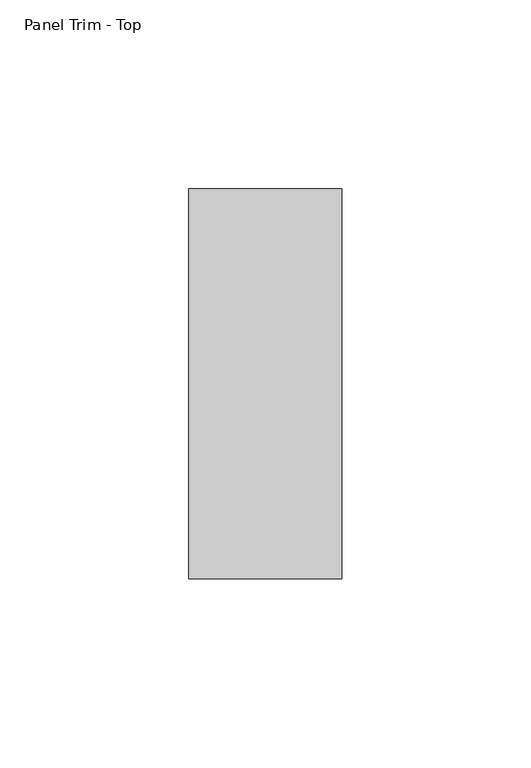
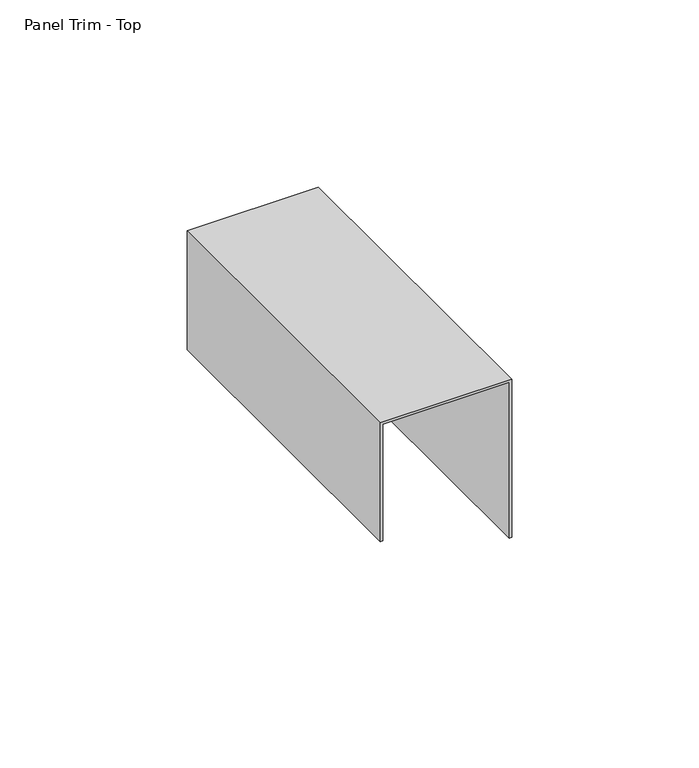
"""IFC4 building model written with IfcOpenShell, lengths in millimetres: proxy geometry, Top Trim - Center Mull : Panel Trim - Top."""

from ifc_helpers import new_model, si_unit, frame, origin, place, context, project, spatial, polyline, outline, extrude, source, transform, mapped, element, save


def panel_trim_top_1c944f5c(model_context):
    return source(origin(), model_context, "Body", "SweptSolid", [
        extrude(outline(polyline([(2438.4, 587327.0060739), (2438.4, 587365.8934739), (2387.6, 587365.8934739), (2387.6, 587366.6808739), (2439.19375, 587366.6808739), (2439.19375, 587326.2186739), (2400.3, 587326.2186739), (2400.3, 587327.0060739), (2438.4, 587327.0060739)])), frame((0.0, -534097.4537841, 0.0), z_axis=(0.0, 1.0, 0.0), x_axis=(0.0, 0.0, 1.0)), (0.0, 0.0, 1.0), 103.1748),
    ])


if __name__ == "__main__":
    model = new_model("IFC4")
    model_context = context("Model", 3, world=origin())
    ifc_project = project(units=[si_unit("LENGTHUNIT", "METRE", prefix="MILLI")], contexts=[model_context])
    site = spatial("IfcSite", under=ifc_project)
    building = spatial("IfcBuilding", under=site)
    placement = place(None, origin())
    panel_trim_top_shape = panel_trim_top_1c944f5c(model_context)
    element("IfcBuildingElementProxy", 1, Name="Top Trim - Center Mull : Panel Trim - Top", ObjectType="Top Trim - Center Mull : Panel Trim - Top", at=placement, inside=building, context=model_context, shape_type="MappedRepresentation", body=[
        mapped(panel_trim_top_shape, transform((0.0, 0.0, 0.0), x_axis=(1.0, 0.0, 0.0), y_axis=(0.0, 1.0, 0.0), z_axis=(0.0, 0.0, 1.0))),
    ])
    save(model, "model.ifc")

# Revit data of these elements
# Element 1 (IfcBuildingElementProxy, "Top Trim - Center Mull : Panel Trim - Top")
#   Materials on its faces: "EDGE TRIM BY MTL PANEL MFR."
# Materials
#   "EDGE TRIM BY MTL PANEL MFR.": class "Generic", colour RGB 239 242 240, transparency 0, Cost = 0
